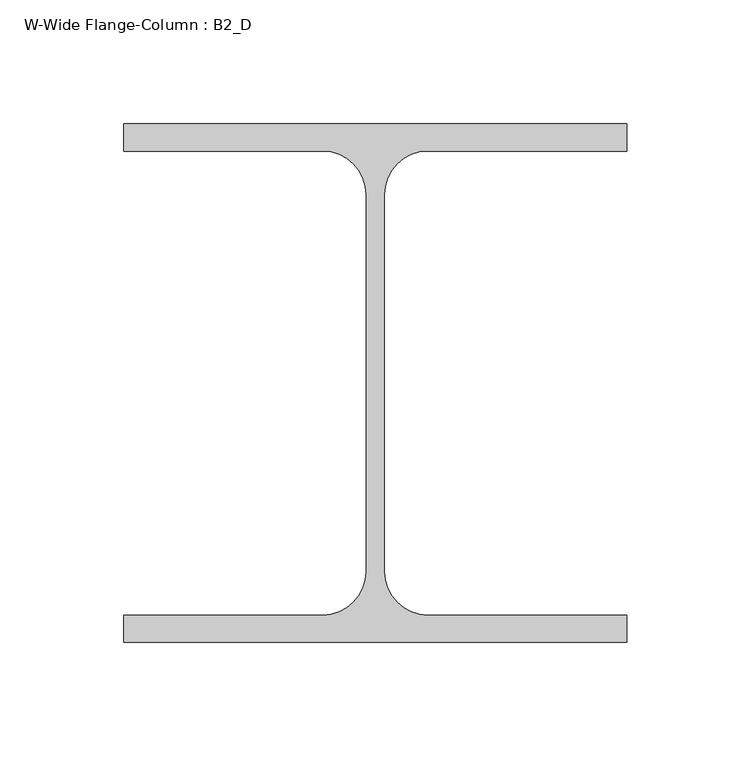
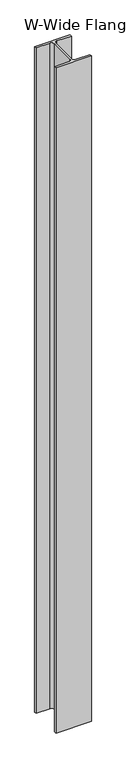
"""IFC4 building model written with IfcOpenShell, lengths in millimetres: column geometry, W-Wide Flange-Column : B2_D."""

import ifcopenshell
import ifcopenshell.guid

model = None  # the IFC model being written
_history = None  # IfcOwnerHistory: only IFC2X3 demands one
_inside = {}  # id of a spatial element -> (the spatial element, [elements in it])
_under = {}  # id of a project, library or spatial element -> (it, [spatial elements below it])
_declared = {}  # id of a project -> (the project, [libraries it declares])
_typed = {}  # id of a type object -> (the type object, [elements of that type])
_made_of = {}  # id of a material, layer set ... -> (it, [elements and type objects made of it])


def new_model(schema):
    """Start an empty IFC model of exactly this schema.

    Asked for "IFC4X3", IfcOpenShell would pick the latest addendum, in which some entities
    have other attributes; the version numbers below select the first issue.
    IFC2X3 requires an IfcOwnerHistory on every rooted entity: one is made here for all.
    """
    global model, _history
    if schema == "IFC4X3":
        model = ifcopenshell.file(schema_version=(4, 3, 0, 0))
    else:
        model = ifcopenshell.file(schema=schema)
    _inside.clear()
    _under.clear()
    _declared.clear()
    _typed.clear()
    _made_of.clear()
    _history = None
    if model.schema == "IFC2X3":
        org = make("IfcOrganization", Name="unknown")
        user = make(
            "IfcPersonAndOrganization",
            ThePerson=make("IfcPerson", FamilyName="unknown"),
            TheOrganization=org,
        )
        app = make(
            "IfcApplication",
            ApplicationDeveloper=org,
            Version="unknown",
            ApplicationFullName="unknown",
            ApplicationIdentifier="unknown",
        )
        _history = make(
            "IfcOwnerHistory",
            OwningUser=user,
            OwningApplication=app,
            ChangeAction="ADDED",
            CreationDate=0,
        )
    return model


def make(cls, **values):
    """One entity of the class cls with the attributes given. An attribute that is None is left unset."""
    return model.create_entity(
        cls, **{name: value for name, value in values.items() if value is not None}
    )


def rooted(cls, **values):
    """An entity with a GlobalId (a new one), such as an element, a storey or a relation."""
    return make(cls, GlobalId=ifcopenshell.guid.new(), OwnerHistory=_history, **values)


def si_unit(unit_type, name, prefix=None):
    """IfcSIUnit, for example si_unit("LENGTHUNIT", "METRE", prefix="MILLI")."""
    return make("IfcSIUnit", UnitType=unit_type, Prefix=prefix, Name=name)


def assignment(units):
    """IfcUnitAssignment: the units of a project."""
    return None if units is None else make("IfcUnitAssignment", Units=units)


def point(xyz):
    """IfcCartesianPoint."""
    return None if xyz is None else make("IfcCartesianPoint", Coordinates=xyz)


def direction(xyz):
    """IfcDirection."""
    return None if xyz is None else make("IfcDirection", DirectionRatios=xyz)


def frame(location, z_axis=None, x_axis=None):
    """IfcAxis2Placement3D, a coordinate frame: its origin and axes. An axis left out is left unset."""
    return make(
        "IfcAxis2Placement3D",
        Location=point(location),
        Axis=direction(z_axis),
        RefDirection=direction(x_axis),
    )


def frame_2d(location, x_axis=None):
    """IfcAxis2Placement2D, a coordinate frame in the plane: its origin and x axis."""
    return make(
        "IfcAxis2Placement2D", Location=point(location), RefDirection=direction(x_axis)
    )


def origin():
    """The frame at (0, 0, 0) with its axes left unset."""
    return frame((0.0, 0.0, 0.0))


def place(relative_to, where):
    """IfcLocalPlacement: puts the frame where relative to a parent placement (None: the world)."""
    return make(
        "IfcLocalPlacement", PlacementRelTo=relative_to, RelativePlacement=where
    )


def context(
    kind, dimensions, precision=None, world=None, true_north=None, identifier=None
):
    """IfcGeometricRepresentationContext, for example the 3D "Model" context."""
    return make(
        "IfcGeometricRepresentationContext",
        ContextIdentifier=identifier,
        ContextType=kind,
        CoordinateSpaceDimension=dimensions,
        Precision=precision,
        WorldCoordinateSystem=world,
        TrueNorth=true_north,
    )


def project(units=None, contexts=None):
    """IfcProject with its units and contexts."""
    return rooted(
        "IfcProject",
        Name="project",
        RepresentationContexts=contexts,
        UnitsInContext=assignment(units),
    )


def spatial(cls, under=None, at=None, **own):
    """A site, building, storey or space (cls), placed at a placement, below another one or the project."""
    s = rooted(cls, ObjectPlacement=at, **own)
    if under is not None:
        _under.setdefault(under.id(), (under, []))[1].append(s)
    return s


def polyline(points):
    """IfcPolyline through the points."""
    return make("IfcPolyline", Points=[point(p) for p in points])


def circle_curve(where, radius):
    """IfcCircle in the frame where."""
    return make("IfcCircle", Position=where, Radius=radius)


def trimmed(basis, trim1, trim2, sense, master):
    """IfcTrimmedCurve: the piece of a basis curve between two trims."""
    return make(
        "IfcTrimmedCurve",
        BasisCurve=basis,
        Trim1=trim1,
        Trim2=trim2,
        SenseAgreement=sense,
        MasterRepresentation=master,
    )


def segment(curve, same_sense, transition):
    """IfcCompositeCurveSegment."""
    return make(
        "IfcCompositeCurveSegment",
        Transition=transition,
        SameSense=same_sense,
        ParentCurve=curve,
    )


def composite_curve(segments, self_intersect=None):
    """IfcCompositeCurve: segments joined end to end."""
    return make("IfcCompositeCurve", Segments=segments, SelfIntersect=self_intersect)


def outline(outer, holes=None, kind="AREA"):
    """IfcArbitraryClosedProfileDef: a profile drawn as a closed curve; with holes, ...WithVoids."""
    if holes is None:
        return make("IfcArbitraryClosedProfileDef", ProfileType=kind, OuterCurve=outer)
    return make(
        "IfcArbitraryProfileDefWithVoids",
        ProfileType=kind,
        OuterCurve=outer,
        InnerCurves=holes,
    )


def extrude(swept, where, along, depth):
    """IfcExtrudedAreaSolid: the profile swept, set in the frame where, extruded along a direction by depth."""
    return make(
        "IfcExtrudedAreaSolid",
        SweptArea=swept,
        Position=where,
        ExtrudedDirection=direction(along),
        Depth=depth,
    )


def shape(context_of_items, identifier, shape_type, items):
    """IfcShapeRepresentation: the items that make up one representation, for example the "Body"."""
    return make(
        "IfcShapeRepresentation",
        ContextOfItems=context_of_items,
        RepresentationIdentifier=identifier,
        RepresentationType=shape_type,
        Items=items,
    )


def source(mapping_origin, context_of_items, identifier, shape_type, items):
    """IfcRepresentationMap: a shape defined once, which mapped items show again and again."""
    return make(
        "IfcRepresentationMap",
        MappingOrigin=mapping_origin,
        MappedRepresentation=shape(context_of_items, identifier, shape_type, items),
    )


def transform(
    local_origin,
    x_axis=None,
    y_axis=None,
    z_axis=None,
    scale=None,
    scale2=None,
    scale3=None,
    uniform=True,
):
    """IfcCartesianTransformationOperator3D, or its non-uniform kind. x_axis, y_axis, z_axis: its Axis1, 2, 3."""
    if uniform:
        return make(
            "IfcCartesianTransformationOperator3D",
            Axis1=direction(x_axis),
            Axis2=direction(y_axis),
            LocalOrigin=point(local_origin),
            Scale=scale,
            Axis3=direction(z_axis),
        )
    return make(
        "IfcCartesianTransformationOperator3DnonUniform",
        Axis1=direction(x_axis),
        Axis2=direction(y_axis),
        LocalOrigin=point(local_origin),
        Scale=scale,
        Axis3=direction(z_axis),
        Scale2=scale2,
        Scale3=scale3,
    )


def mapped(mapping_source, mapping_target):
    """IfcMappedItem: shows the shape of a source again, moved by a transform."""
    return make(
        "IfcMappedItem", MappingSource=mapping_source, MappingTarget=mapping_target
    )


def made_of(thing, what):
    """Note that an element or type object is made of a material, layer set ...; save() writes the relation."""
    if what is not None:
        _made_of.setdefault(what.id(), (what, []))[1].append(thing)
    return thing


def element(
    cls,
    number,
    at=None,
    inside=None,
    cuts=None,
    type_object=None,
    material=None,
    context=None,
    identifier="Body",
    shape_type=None,
    held_by="IfcProductDefinitionShape",
    body=None,
    shapes=None,
    **own,
):
    """One element of the class cls, such as IfcWall. Its Tag is "e" and its number.

    at: its placement. inside: the storey or other place that contains it. cuts: it is an
    opening in that element (IfcRelVoidsElement). A single representation is given by context,
    identifier, shape_type and body (its items); several are given by shapes. held_by: the class
    of the entity that holds the representations. save() writes the other relations.
    """
    e = rooted(cls, Tag="e%d" % number, ObjectPlacement=at, **own)
    if body is not None:
        shapes = [shape(context, identifier, shape_type, body)]
    if shapes is not None:
        e.Representation = make(held_by, Representations=shapes)
    if inside is not None:
        _inside.setdefault(inside.id(), (inside, []))[1].append(e)
    if cuts is not None:
        rooted(
            "IfcRelVoidsElement", RelatingBuildingElement=cuts, RelatedOpeningElement=e
        )
    if type_object is not None:
        _typed.setdefault(type_object.id(), (type_object, []))[1].append(e)
    return made_of(e, material)


def aggregate(whole, parts):
    """IfcRelAggregates: a whole, such as a stair, and the parts it consists of."""
    return rooted("IfcRelAggregates", RelatingObject=whole, RelatedObjects=parts)


def save(model, path):
    """Write the relations noted so far, then the file.

    IfcRelAggregates (storeys below a building ...), IfcRelContainedInSpatialStructure (elements
    in a storey), IfcRelDefinesByType, IfcRelAssociatesMaterial and IfcRelDeclares: one each for
    every whole, place, type object, material and project.
    """
    for whole, parts in _under.values():
        aggregate(whole, parts)
    for where, things in _inside.values():
        rooted(
            "IfcRelContainedInSpatialStructure",
            RelatedElements=things,
            RelatingStructure=where,
        )
    for kind, things in _typed.values():
        rooted("IfcRelDefinesByType", RelatedObjects=things, RelatingType=kind)
    for what, things in _made_of.values():
        rooted("IfcRelAssociatesMaterial", RelatedObjects=things, RelatingMaterial=what)
    for by, libraries in _declared.values():
        rooted("IfcRelDeclares", RelatingContext=by, RelatedDefinitions=libraries)
    model.write(path)


def w_wide_flange_column_b2_d_8d82b8b8(model_context):
    return source(origin(), model_context, "Body", "SweptSolid", [
        extrude(outline(composite_curve([segment(polyline([(101.6, 104.775), (101.6, 93.7617188), (21.2328125, 93.7617188)]), True, "CONTINUOUS"), segment(trimmed(circle_curve(frame_2d((21.2328125, 76.2)), 17.5617188), [point((21.2328125, 93.7617188))], [point((3.6710937, 76.2))], True, "CARTESIAN"), True, "CONTINUOUS"), segment(polyline([(3.6710937, 76.2), (3.6710937, -76.2)]), True, "CONTINUOUS"), segment(trimmed(circle_curve(frame_2d((21.2328125, -76.2)), 17.5617188), [point((3.6710937, -76.2))], [point((21.2328125, -93.7617187))], True, "CARTESIAN"), True, "CONTINUOUS"), segment(polyline([(21.2328125, -93.7617187), (101.6, -93.7617187), (101.6, -104.775), (-101.6, -104.775), (-101.6, -93.7617187), (-21.2328125, -93.7617187)]), True, "CONTINUOUS"), segment(trimmed(circle_curve(frame_2d((-21.2328125, -76.2)), 17.5617188), [point((-21.2328125, -93.7617187))], [point((-3.6710938, -76.2))], True, "CARTESIAN"), True, "CONTINUOUS"), segment(polyline([(-3.6710938, -76.2), (-3.6710938, 76.2)]), True, "CONTINUOUS"), segment(trimmed(circle_curve(frame_2d((-21.2328125, 76.2)), 17.5617188), [point((-3.6710938, 76.2))], [point((-21.2328125, 93.7617188))], True, "CARTESIAN"), True, "CONTINUOUS"), segment(polyline([(-21.2328125, 93.7617188), (-101.6, 93.7617188), (-101.6, 104.775), (101.6, 104.775)]), True, "CONTINUOUS")], self_intersect=False)), frame((0.0, 0.0, -304.8), z_axis=(0.0, 0.0, 1.0), x_axis=(1.0, 0.0, 0.0)), (0.0, 0.0, 1.0), 4025.9),
    ])


if __name__ == "__main__":
    model = new_model("IFC4")
    model_context = context("Model", 3, world=origin())
    ifc_project = project(units=[si_unit("LENGTHUNIT", "METRE", prefix="MILLI")], contexts=[model_context])
    site = spatial("IfcSite", under=ifc_project)
    building = spatial("IfcBuilding", under=site)
    placement = place(None, origin())
    w_wide_flange_column_b2_d_shape = w_wide_flange_column_b2_d_8d82b8b8(model_context)
    element("IfcColumn", 1, ObjectType="W-Wide Flange-Column : B2_D", at=placement, inside=building, context=model_context, shape_type="MappedRepresentation", body=[
        mapped(w_wide_flange_column_b2_d_shape, transform((0.0, 0.0, 0.0), x_axis=(1.0, 0.0, 0.0), y_axis=(0.0, 1.0, 0.0), z_axis=(0.0, 0.0, 1.0))),
    ])
    save(model, "model.ifc")

# Revit data of these elements
# Type "W-Wide Flange-Column : B2_D"
#   Assembly Code = "B10"
#   W = 33
#   bf = 0' - 8"
#   d = 0' - 8 1/4"
#   k = 0' - 1 1/8"
#   kr = 0' - 0 177/256"
#   tf = 0' - 0 111/256"
#   tw = 0' - 0 37/128"
#   A = 0.07 SF
#   Structural Material [instance default] = Steel ASTM A992
# Element 1 (IfcColumn, "W-Wide Flange-Column : B2_D")
#   Structural Material = STRUCTURAL STEEL - SEE STRUCT. DWGS
#   Materials on its faces: "STRUCTURAL STEEL - SEE STRUCT. DWGS"
# Materials
#   "Steel ASTM A992": class "Metal", colour RGB 199 199 199, transparency 0, Description = "Structural steel 50ksi", Cost = 0
#   "STRUCTURAL STEEL - SEE STRUCT. DWGS": class "Metal", colour RGB 137 146 153, transparency 0, Description = "Steel, mill finish", Cost = 0
